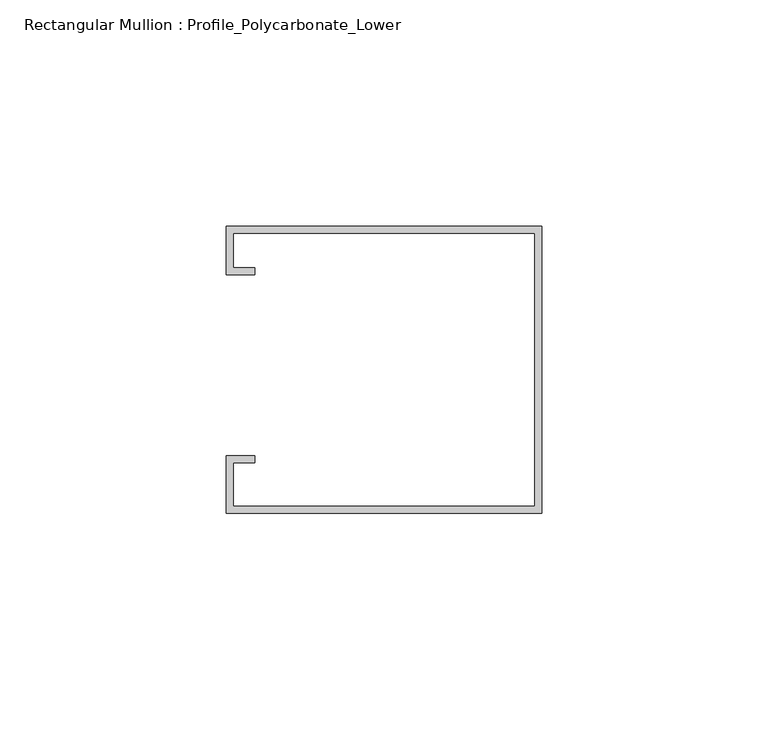
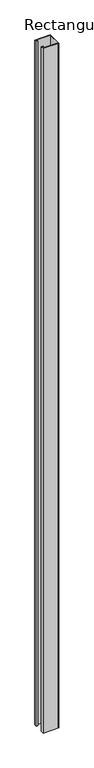
"""IFC4 building model written with IfcOpenShell, lengths in millimetres: member geometry, Rectangular Mullion : Profile_Polycarbonate_Lower."""

import ifcopenshell
import ifcopenshell.guid

model = None  # the IFC model being written
_history = None  # IfcOwnerHistory: only IFC2X3 demands one
_inside = {}  # id of a spatial element -> (the spatial element, [elements in it])
_under = {}  # id of a project, library or spatial element -> (it, [spatial elements below it])
_declared = {}  # id of a project -> (the project, [libraries it declares])
_typed = {}  # id of a type object -> (the type object, [elements of that type])
_made_of = {}  # id of a material, layer set ... -> (it, [elements and type objects made of it])


def new_model(schema):
    """Start an empty IFC model of exactly this schema.

    Asked for "IFC4X3", IfcOpenShell would pick the latest addendum, in which some entities
    have other attributes; the version numbers below select the first issue.
    IFC2X3 requires an IfcOwnerHistory on every rooted entity: one is made here for all.
    """
    global model, _history
    if schema == "IFC4X3":
        model = ifcopenshell.file(schema_version=(4, 3, 0, 0))
    else:
        model = ifcopenshell.file(schema=schema)
    _inside.clear()
    _under.clear()
    _declared.clear()
    _typed.clear()
    _made_of.clear()
    _history = None
    if model.schema == "IFC2X3":
        org = make("IfcOrganization", Name="unknown")
        user = make(
            "IfcPersonAndOrganization",
            ThePerson=make("IfcPerson", FamilyName="unknown"),
            TheOrganization=org,
        )
        app = make(
            "IfcApplication",
            ApplicationDeveloper=org,
            Version="unknown",
            ApplicationFullName="unknown",
            ApplicationIdentifier="unknown",
        )
        _history = make(
            "IfcOwnerHistory",
            OwningUser=user,
            OwningApplication=app,
            ChangeAction="ADDED",
            CreationDate=0,
        )
    return model


def make(cls, **values):
    """One entity of the class cls with the attributes given. An attribute that is None is left unset."""
    return model.create_entity(
        cls, **{name: value for name, value in values.items() if value is not None}
    )


def rooted(cls, **values):
    """An entity with a GlobalId (a new one), such as an element, a storey or a relation."""
    return make(cls, GlobalId=ifcopenshell.guid.new(), OwnerHistory=_history, **values)


def si_unit(unit_type, name, prefix=None):
    """IfcSIUnit, for example si_unit("LENGTHUNIT", "METRE", prefix="MILLI")."""
    return make("IfcSIUnit", UnitType=unit_type, Prefix=prefix, Name=name)


def assignment(units):
    """IfcUnitAssignment: the units of a project."""
    return None if units is None else make("IfcUnitAssignment", Units=units)


def point(xyz):
    """IfcCartesianPoint."""
    return None if xyz is None else make("IfcCartesianPoint", Coordinates=xyz)


def direction(xyz):
    """IfcDirection."""
    return None if xyz is None else make("IfcDirection", DirectionRatios=xyz)


def frame(location, z_axis=None, x_axis=None):
    """IfcAxis2Placement3D, a coordinate frame: its origin and axes. An axis left out is left unset."""
    return make(
        "IfcAxis2Placement3D",
        Location=point(location),
        Axis=direction(z_axis),
        RefDirection=direction(x_axis),
    )


def origin():
    """The frame at (0, 0, 0) with its axes left unset."""
    return frame((0.0, 0.0, 0.0))


def place(relative_to, where):
    """IfcLocalPlacement: puts the frame where relative to a parent placement (None: the world)."""
    return make(
        "IfcLocalPlacement", PlacementRelTo=relative_to, RelativePlacement=where
    )


def context(
    kind, dimensions, precision=None, world=None, true_north=None, identifier=None
):
    """IfcGeometricRepresentationContext, for example the 3D "Model" context."""
    return make(
        "IfcGeometricRepresentationContext",
        ContextIdentifier=identifier,
        ContextType=kind,
        CoordinateSpaceDimension=dimensions,
        Precision=precision,
        WorldCoordinateSystem=world,
        TrueNorth=true_north,
    )


def project(units=None, contexts=None):
    """IfcProject with its units and contexts."""
    return rooted(
        "IfcProject",
        Name="project",
        RepresentationContexts=contexts,
        UnitsInContext=assignment(units),
    )


def spatial(cls, under=None, at=None, **own):
    """A site, building, storey or space (cls), placed at a placement, below another one or the project."""
    s = rooted(cls, ObjectPlacement=at, **own)
    if under is not None:
        _under.setdefault(under.id(), (under, []))[1].append(s)
    return s


def polyline(points):
    """IfcPolyline through the points."""
    return make("IfcPolyline", Points=[point(p) for p in points])


def outline(outer, holes=None, kind="AREA"):
    """IfcArbitraryClosedProfileDef: a profile drawn as a closed curve; with holes, ...WithVoids."""
    if holes is None:
        return make("IfcArbitraryClosedProfileDef", ProfileType=kind, OuterCurve=outer)
    return make(
        "IfcArbitraryProfileDefWithVoids",
        ProfileType=kind,
        OuterCurve=outer,
        InnerCurves=holes,
    )


def extrude(swept, where, along, depth):
    """IfcExtrudedAreaSolid: the profile swept, set in the frame where, extruded along a direction by depth."""
    return make(
        "IfcExtrudedAreaSolid",
        SweptArea=swept,
        Position=where,
        ExtrudedDirection=direction(along),
        Depth=depth,
    )


def shape(context_of_items, identifier, shape_type, items):
    """IfcShapeRepresentation: the items that make up one representation, for example the "Body"."""
    return make(
        "IfcShapeRepresentation",
        ContextOfItems=context_of_items,
        RepresentationIdentifier=identifier,
        RepresentationType=shape_type,
        Items=items,
    )


def source(mapping_origin, context_of_items, identifier, shape_type, items):
    """IfcRepresentationMap: a shape defined once, which mapped items show again and again."""
    return make(
        "IfcRepresentationMap",
        MappingOrigin=mapping_origin,
        MappedRepresentation=shape(context_of_items, identifier, shape_type, items),
    )


def transform(
    local_origin,
    x_axis=None,
    y_axis=None,
    z_axis=None,
    scale=None,
    scale2=None,
    scale3=None,
    uniform=True,
):
    """IfcCartesianTransformationOperator3D, or its non-uniform kind. x_axis, y_axis, z_axis: its Axis1, 2, 3."""
    if uniform:
        return make(
            "IfcCartesianTransformationOperator3D",
            Axis1=direction(x_axis),
            Axis2=direction(y_axis),
            LocalOrigin=point(local_origin),
            Scale=scale,
            Axis3=direction(z_axis),
        )
    return make(
        "IfcCartesianTransformationOperator3DnonUniform",
        Axis1=direction(x_axis),
        Axis2=direction(y_axis),
        LocalOrigin=point(local_origin),
        Scale=scale,
        Axis3=direction(z_axis),
        Scale2=scale2,
        Scale3=scale3,
    )


def mapped(mapping_source, mapping_target):
    """IfcMappedItem: shows the shape of a source again, moved by a transform."""
    return make(
        "IfcMappedItem", MappingSource=mapping_source, MappingTarget=mapping_target
    )


def made_of(thing, what):
    """Note that an element or type object is made of a material, layer set ...; save() writes the relation."""
    if what is not None:
        _made_of.setdefault(what.id(), (what, []))[1].append(thing)
    return thing


def element(
    cls,
    number,
    at=None,
    inside=None,
    cuts=None,
    type_object=None,
    material=None,
    context=None,
    identifier="Body",
    shape_type=None,
    held_by="IfcProductDefinitionShape",
    body=None,
    shapes=None,
    **own,
):
    """One element of the class cls, such as IfcWall. Its Tag is "e" and its number.

    at: its placement. inside: the storey or other place that contains it. cuts: it is an
    opening in that element (IfcRelVoidsElement). A single representation is given by context,
    identifier, shape_type and body (its items); several are given by shapes. held_by: the class
    of the entity that holds the representations. save() writes the other relations.
    """
    e = rooted(cls, Tag="e%d" % number, ObjectPlacement=at, **own)
    if body is not None:
        shapes = [shape(context, identifier, shape_type, body)]
    if shapes is not None:
        e.Representation = make(held_by, Representations=shapes)
    if inside is not None:
        _inside.setdefault(inside.id(), (inside, []))[1].append(e)
    if cuts is not None:
        rooted(
            "IfcRelVoidsElement", RelatingBuildingElement=cuts, RelatedOpeningElement=e
        )
    if type_object is not None:
        _typed.setdefault(type_object.id(), (type_object, []))[1].append(e)
    return made_of(e, material)


def aggregate(whole, parts):
    """IfcRelAggregates: a whole, such as a stair, and the parts it consists of."""
    return rooted("IfcRelAggregates", RelatingObject=whole, RelatedObjects=parts)


def save(model, path):
    """Write the relations noted so far, then the file.

    IfcRelAggregates (storeys below a building ...), IfcRelContainedInSpatialStructure (elements
    in a storey), IfcRelDefinesByType, IfcRelAssociatesMaterial and IfcRelDeclares: one each for
    every whole, place, type object, material and project.
    """
    for whole, parts in _under.values():
        aggregate(whole, parts)
    for where, things in _inside.values():
        rooted(
            "IfcRelContainedInSpatialStructure",
            RelatedElements=things,
            RelatingStructure=where,
        )
    for kind, things in _typed.values():
        rooted("IfcRelDefinesByType", RelatedObjects=things, RelatingType=kind)
    for what, things in _made_of.values():
        rooted("IfcRelAssociatesMaterial", RelatedObjects=things, RelatingMaterial=what)
    for by, libraries in _declared.values():
        rooted("IfcRelDeclares", RelatingContext=by, RelatedDefinitions=libraries)
    model.write(path)


def rectangular_mullion_profile_polycarbonate_lower_31cbd8d6(model_context):
    return source(origin(), model_context, "Body", "SweptSolid", [
        extrude(outline(polyline([(0.0, -32.7), (-69.85, -32.7), (-69.85, -20.0), (-63.5, -20.0), (-63.5, -21.5875), (-68.2625, -21.5875), (-68.2625, -31.1125), (-1.5875, -31.1125), (-1.5875, 29.2125), (-68.2625, 29.2125), (-68.2625, 21.5875), (-63.5, 21.5875), (-63.5, 20.0), (-69.85, 20.0), (-69.85, 30.8), (0.0, 30.8), (0.0, -32.7)])), frame((0.0, 0.0, -3251.2), z_axis=(0.0, 0.0, 1.0), x_axis=(1.0, 0.0, 0.0)), (0.0, 0.0, 1.0), 3251.2),
    ])


if __name__ == "__main__":
    model = new_model("IFC4")
    model_context = context("Model", 3, world=origin())
    ifc_project = project(units=[si_unit("LENGTHUNIT", "METRE", prefix="MILLI")], contexts=[model_context])
    site = spatial("IfcSite", under=ifc_project)
    building = spatial("IfcBuilding", under=site)
    placement = place(None, origin())
    rectangular_mullion_profile_polycarbonate_lower_shape = rectangular_mullion_profile_polycarbonate_lower_31cbd8d6(model_context)
    element("IfcMember", 1, ObjectType="Rectangular Mullion : Profile_Polycarbonate_Lower", at=placement, inside=building, context=model_context, shape_type="MappedRepresentation", body=[
        mapped(rectangular_mullion_profile_polycarbonate_lower_shape, transform((0.0, 0.0, 0.0), x_axis=(1.0, 0.0, 0.0), y_axis=(0.0, 1.0, 0.0), z_axis=(0.0, 0.0, 1.0))),
    ])
    save(model, "model.ifc")

# Revit data of these elements
# Type "Rectangular Mullion : Profile_Polycarbonate_Lower"
#   built-in parameter 1007322 = 0.208333 (stored number, unit not read)
#   built-in parameter 1007321 = 0 (stored number, unit not read)
#   built-in parameter 1007320 = 0.00520833 (stored number, unit not read)
# Element 1 (IfcMember, "Rectangular Mullion : Profile_Polycarbonate_Lower")
#   Materials on its faces: "ALUMINUM PROFILE AT POLYCARBONATE PANEL"
# Materials
#   "ALUMINUM PROFILE AT POLYCARBONATE PANEL": class "Metal", colour RGB 244 244 244, transparency 0, Description = "Aluminum 6061", Cost = 0
